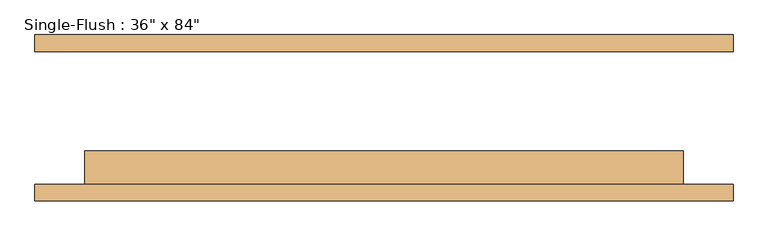
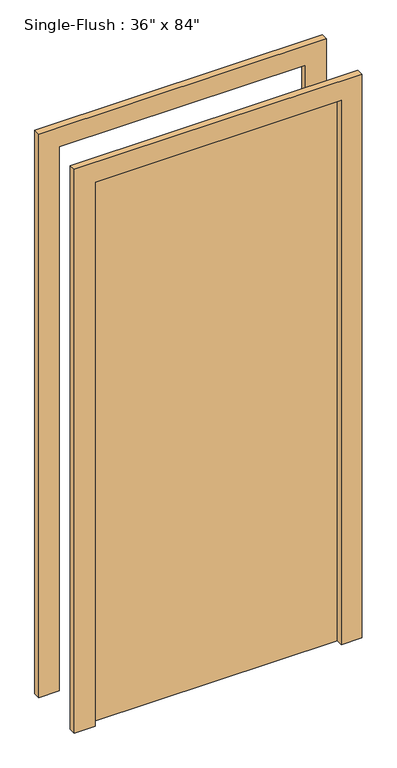
"""IFC4 building model written with IfcOpenShell, lengths in millimetres: door geometry."""

import ifcopenshell
import ifcopenshell.guid

model = None  # the IFC model being written
_history = None  # IfcOwnerHistory: only IFC2X3 demands one
_inside = {}  # id of a spatial element -> (the spatial element, [elements in it])
_under = {}  # id of a project, library or spatial element -> (it, [spatial elements below it])
_declared = {}  # id of a project -> (the project, [libraries it declares])
_typed = {}  # id of a type object -> (the type object, [elements of that type])
_made_of = {}  # id of a material, layer set ... -> (it, [elements and type objects made of it])


def new_model(schema):
    """Start an empty IFC model of exactly this schema.

    Asked for "IFC4X3", IfcOpenShell would pick the latest addendum, in which some entities
    have other attributes; the version numbers below select the first issue.
    IFC2X3 requires an IfcOwnerHistory on every rooted entity: one is made here for all.
    """
    global model, _history
    if schema == "IFC4X3":
        model = ifcopenshell.file(schema_version=(4, 3, 0, 0))
    else:
        model = ifcopenshell.file(schema=schema)
    _inside.clear()
    _under.clear()
    _declared.clear()
    _typed.clear()
    _made_of.clear()
    _history = None
    if model.schema == "IFC2X3":
        org = make("IfcOrganization", Name="unknown")
        user = make(
            "IfcPersonAndOrganization",
            ThePerson=make("IfcPerson", FamilyName="unknown"),
            TheOrganization=org,
        )
        app = make(
            "IfcApplication",
            ApplicationDeveloper=org,
            Version="unknown",
            ApplicationFullName="unknown",
            ApplicationIdentifier="unknown",
        )
        _history = make(
            "IfcOwnerHistory",
            OwningUser=user,
            OwningApplication=app,
            ChangeAction="ADDED",
            CreationDate=0,
        )
    return model


def make(cls, **values):
    """One entity of the class cls with the attributes given. An attribute that is None is left unset."""
    return model.create_entity(
        cls, **{name: value for name, value in values.items() if value is not None}
    )


def rooted(cls, **values):
    """An entity with a GlobalId (a new one), such as an element, a storey or a relation."""
    return make(cls, GlobalId=ifcopenshell.guid.new(), OwnerHistory=_history, **values)


def si_unit(unit_type, name, prefix=None):
    """IfcSIUnit, for example si_unit("LENGTHUNIT", "METRE", prefix="MILLI")."""
    return make("IfcSIUnit", UnitType=unit_type, Prefix=prefix, Name=name)


def assignment(units):
    """IfcUnitAssignment: the units of a project."""
    return None if units is None else make("IfcUnitAssignment", Units=units)


def point(xyz):
    """IfcCartesianPoint."""
    return None if xyz is None else make("IfcCartesianPoint", Coordinates=xyz)


def direction(xyz):
    """IfcDirection."""
    return None if xyz is None else make("IfcDirection", DirectionRatios=xyz)


def frame(location, z_axis=None, x_axis=None):
    """IfcAxis2Placement3D, a coordinate frame: its origin and axes. An axis left out is left unset."""
    return make(
        "IfcAxis2Placement3D",
        Location=point(location),
        Axis=direction(z_axis),
        RefDirection=direction(x_axis),
    )


def origin():
    """The frame at (0, 0, 0) with its axes left unset."""
    return frame((0.0, 0.0, 0.0))


def origin_with_axes():
    """The frame at (0, 0, 0) with the z axis (0, 0, 1) and the x axis (1, 0, 0) written out."""
    return frame((0.0, 0.0, 0.0), z_axis=(0.0, 0.0, 1.0), x_axis=(1.0, 0.0, 0.0))


def place(relative_to, where):
    """IfcLocalPlacement: puts the frame where relative to a parent placement (None: the world)."""
    return make(
        "IfcLocalPlacement", PlacementRelTo=relative_to, RelativePlacement=where
    )


def context(
    kind, dimensions, precision=None, world=None, true_north=None, identifier=None
):
    """IfcGeometricRepresentationContext, for example the 3D "Model" context."""
    return make(
        "IfcGeometricRepresentationContext",
        ContextIdentifier=identifier,
        ContextType=kind,
        CoordinateSpaceDimension=dimensions,
        Precision=precision,
        WorldCoordinateSystem=world,
        TrueNorth=true_north,
    )


def project(units=None, contexts=None):
    """IfcProject with its units and contexts."""
    return rooted(
        "IfcProject",
        Name="project",
        RepresentationContexts=contexts,
        UnitsInContext=assignment(units),
    )


def spatial(cls, under=None, at=None, **own):
    """A site, building, storey or space (cls), placed at a placement, below another one or the project."""
    s = rooted(cls, ObjectPlacement=at, **own)
    if under is not None:
        _under.setdefault(under.id(), (under, []))[1].append(s)
    return s


def polyline(points):
    """IfcPolyline through the points."""
    return make("IfcPolyline", Points=[point(p) for p in points])


def outline(outer, holes=None, kind="AREA"):
    """IfcArbitraryClosedProfileDef: a profile drawn as a closed curve; with holes, ...WithVoids."""
    if holes is None:
        return make("IfcArbitraryClosedProfileDef", ProfileType=kind, OuterCurve=outer)
    return make(
        "IfcArbitraryProfileDefWithVoids",
        ProfileType=kind,
        OuterCurve=outer,
        InnerCurves=holes,
    )


def extrude(swept, where, along, depth):
    """IfcExtrudedAreaSolid: the profile swept, set in the frame where, extruded along a direction by depth."""
    return make(
        "IfcExtrudedAreaSolid",
        SweptArea=swept,
        Position=where,
        ExtrudedDirection=direction(along),
        Depth=depth,
    )


def shape(context_of_items, identifier, shape_type, items):
    """IfcShapeRepresentation: the items that make up one representation, for example the "Body"."""
    return make(
        "IfcShapeRepresentation",
        ContextOfItems=context_of_items,
        RepresentationIdentifier=identifier,
        RepresentationType=shape_type,
        Items=items,
    )


def source(mapping_origin, context_of_items, identifier, shape_type, items):
    """IfcRepresentationMap: a shape defined once, which mapped items show again and again."""
    return make(
        "IfcRepresentationMap",
        MappingOrigin=mapping_origin,
        MappedRepresentation=shape(context_of_items, identifier, shape_type, items),
    )


def transform(
    local_origin,
    x_axis=None,
    y_axis=None,
    z_axis=None,
    scale=None,
    scale2=None,
    scale3=None,
    uniform=True,
):
    """IfcCartesianTransformationOperator3D, or its non-uniform kind. x_axis, y_axis, z_axis: its Axis1, 2, 3."""
    if uniform:
        return make(
            "IfcCartesianTransformationOperator3D",
            Axis1=direction(x_axis),
            Axis2=direction(y_axis),
            LocalOrigin=point(local_origin),
            Scale=scale,
            Axis3=direction(z_axis),
        )
    return make(
        "IfcCartesianTransformationOperator3DnonUniform",
        Axis1=direction(x_axis),
        Axis2=direction(y_axis),
        LocalOrigin=point(local_origin),
        Scale=scale,
        Axis3=direction(z_axis),
        Scale2=scale2,
        Scale3=scale3,
    )


def mapped(mapping_source, mapping_target):
    """IfcMappedItem: shows the shape of a source again, moved by a transform."""
    return make(
        "IfcMappedItem", MappingSource=mapping_source, MappingTarget=mapping_target
    )


def made_of(thing, what):
    """Note that an element or type object is made of a material, layer set ...; save() writes the relation."""
    if what is not None:
        _made_of.setdefault(what.id(), (what, []))[1].append(thing)
    return thing


def element(
    cls,
    number,
    at=None,
    inside=None,
    cuts=None,
    type_object=None,
    material=None,
    context=None,
    identifier="Body",
    shape_type=None,
    held_by="IfcProductDefinitionShape",
    body=None,
    shapes=None,
    **own,
):
    """One element of the class cls, such as IfcWall. Its Tag is "e" and its number.

    at: its placement. inside: the storey or other place that contains it. cuts: it is an
    opening in that element (IfcRelVoidsElement). A single representation is given by context,
    identifier, shape_type and body (its items); several are given by shapes. held_by: the class
    of the entity that holds the representations. save() writes the other relations.
    """
    e = rooted(cls, Tag="e%d" % number, ObjectPlacement=at, **own)
    if body is not None:
        shapes = [shape(context, identifier, shape_type, body)]
    if shapes is not None:
        e.Representation = make(held_by, Representations=shapes)
    if inside is not None:
        _inside.setdefault(inside.id(), (inside, []))[1].append(e)
    if cuts is not None:
        rooted(
            "IfcRelVoidsElement", RelatingBuildingElement=cuts, RelatedOpeningElement=e
        )
    if type_object is not None:
        _typed.setdefault(type_object.id(), (type_object, []))[1].append(e)
    return made_of(e, material)


def aggregate(whole, parts):
    """IfcRelAggregates: a whole, such as a stair, and the parts it consists of."""
    return rooted("IfcRelAggregates", RelatingObject=whole, RelatedObjects=parts)


def save(model, path):
    """Write the relations noted so far, then the file.

    IfcRelAggregates (storeys below a building ...), IfcRelContainedInSpatialStructure (elements
    in a storey), IfcRelDefinesByType, IfcRelAssociatesMaterial and IfcRelDeclares: one each for
    every whole, place, type object, material and project.
    """
    for whole, parts in _under.values():
        aggregate(whole, parts)
    for where, things in _inside.values():
        rooted(
            "IfcRelContainedInSpatialStructure",
            RelatedElements=things,
            RelatingStructure=where,
        )
    for kind, things in _typed.values():
        rooted("IfcRelDefinesByType", RelatedObjects=things, RelatingType=kind)
    for what, things in _made_of.values():
        rooted("IfcRelAssociatesMaterial", RelatedObjects=things, RelatingMaterial=what)
    for by, libraries in _declared.values():
        rooted("IfcRelDeclares", RelatingContext=by, RelatedDefinitions=libraries)
    model.write(path)


def door_719f80de(model_context):
    return source(origin(), model_context, "Body", "SweptSolid", [
        extrude(outline(polyline([(2209.8, -533.4), (0.0, -533.4), (0.0, -457.2), (2133.6, -457.2), (2133.6, 457.2), (0.0, 457.2), (0.0, 533.4), (2209.8, 533.4), (2209.8, -533.4)])), frame((0.0, -127.0, 0.0), z_axis=(0.0, 1.0, 0.0), x_axis=(0.0, 0.0, 1.0)), (0.0, 0.0, 1.0), 25.4),
        extrude(outline(polyline([(2209.8, 533.4), (2209.8, -533.4), (0.0, -533.4), (0.0, -457.2), (2133.6, -457.2), (2133.6, 457.2), (0.0, 457.2), (0.0, 533.4), (2209.8, 533.4)])), frame((0.0, 101.6, 0.0), z_axis=(0.0, 1.0, 0.0), x_axis=(0.0, 0.0, 1.0)), (0.0, 0.0, 1.0), 25.4),
        extrude(outline(polyline([(457.2, -50.8), (457.2, -101.6), (-457.2, -101.6), (-457.2, -50.8), (457.2, -50.8)])), origin_with_axes(), (0.0, 0.0, 1.0), 2133.6),
    ])


if __name__ == "__main__":
    model = new_model("IFC4")
    model_context = context("Model", 3, world=origin())
    ifc_project = project(units=[si_unit("LENGTHUNIT", "METRE", prefix="MILLI")], contexts=[model_context])
    site = spatial("IfcSite", under=ifc_project)
    building = spatial("IfcBuilding", under=site)
    placement = place(None, origin())
    door_shape = door_719f80de(model_context)
    element("IfcDoor", 1, ObjectType="Single-Flush : 36\" x 84\"", at=placement, inside=building, context=model_context, shape_type="MappedRepresentation", body=[
        mapped(door_shape, transform((0.0, 0.0, 0.0), x_axis=(1.0, 0.0, 0.0), y_axis=(0.0, 1.0, 0.0), z_axis=(0.0, 0.0, 1.0))),
    ])
    save(model, "model.ifc")

# Revit data of these elements
# Type "Single-Flush : 36\" x 84\""
#   Type Mark = "34"
#   Assembly Code = "C1020"
#   Thickness = 0' - 2"
#   Height = 7' - 0"
#   Trim Projection Ext = 0' - 1"
#   Trim Projection Int = 0' - 1"
#   Trim Width = 0' - 3"
#   Width = 3' - 0"
#   Define Thermal Properties by = 0
#   Function = 0
#   Door Material = Door - Panel
#   Frame Material = Door - Frame
#   Wall Closure = (empty or 0)
# Element 1 (IfcDoor, "Single-Flush : 36\" x 84\"")
#   Materials on its faces: "Door - Frame", "Door - Panel"
# Materials
#   "Door - Panel": class "Wood", colour RGB 227 170 128, transparency 0, Cost = 0
#   "Door - Frame": class "Miscellaneous", colour RGB 153 76 43, transparency 0, Cost = 0
